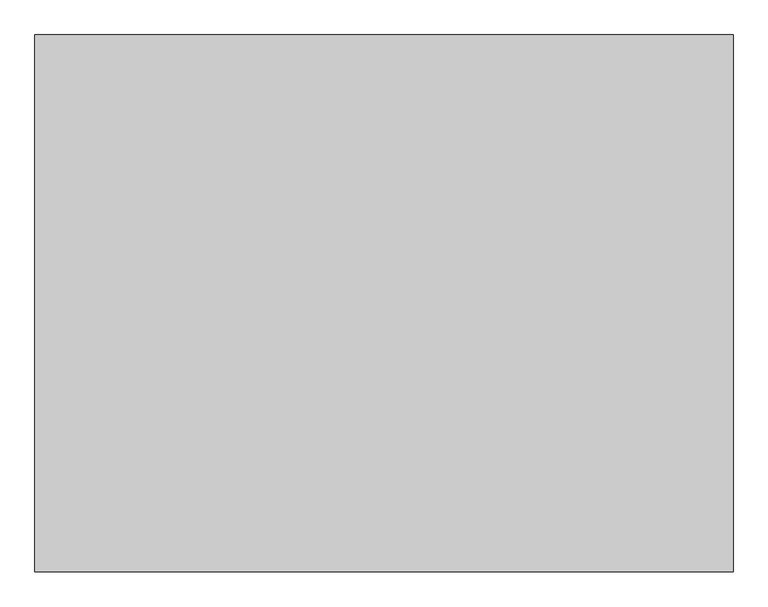
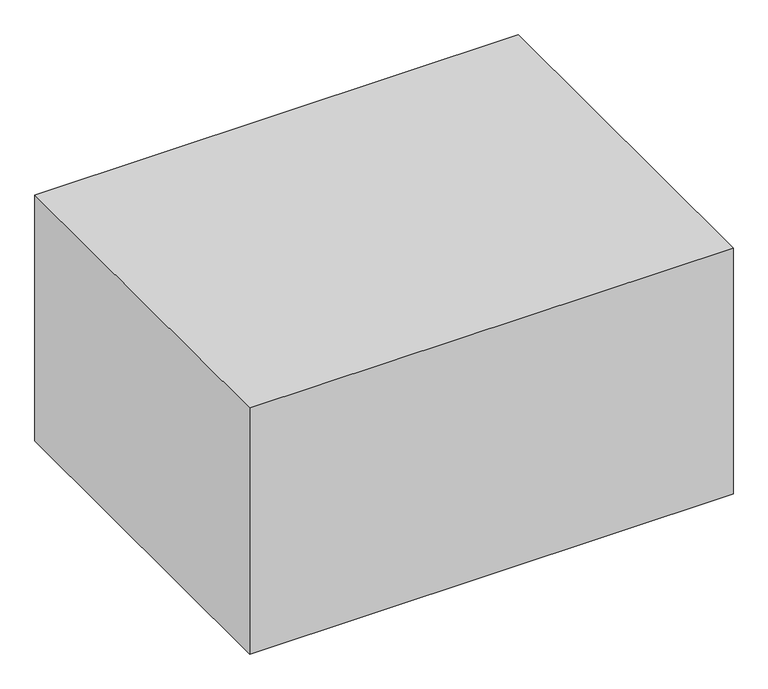
"""IFC4 building model written with IfcOpenShell, lengths in millimetres: proxy geometry, Space Planning Box_hec : Space Planning Box_hec."""

from ifc_helpers import new_model, si_unit, origin, origin_with_axes, place, context, project, spatial, polyline, outline, extrude, source, transform, mapped, element, save


def generic_models_249c6621(model_context):
    return source(origin(), model_context, "Body", "SweptSolid", [
        extrude(outline(polyline([(3250.0, 2500.0), (3250.0, -2500.0), (-3250.0, -2500.0), (-3250.0, 2500.0), (3250.0, 2500.0)])), origin_with_axes(), (0.0, 0.0, 1.0), 3500.0),
    ])


if __name__ == "__main__":
    model = new_model("IFC4")
    model_context = context("Model", 3, world=origin())
    ifc_project = project(units=[si_unit("LENGTHUNIT", "METRE", prefix="MILLI")], contexts=[model_context])
    site = spatial("IfcSite", under=ifc_project)
    building = spatial("IfcBuilding", under=site)
    placement = place(None, origin())
    generic_models_shape = generic_models_249c6621(model_context)
    element("IfcBuildingElementProxy", 1, Name="Space Planning Box_hec : Space Planning Box_hec", ObjectType="Space Planning Box_hec : Space Planning Box_hec", at=placement, inside=building, context=model_context, shape_type="MappedRepresentation", body=[
        mapped(generic_models_shape, transform((0.0, 0.0, 0.0), x_axis=(1.0, 0.0, 0.0), y_axis=(0.0, 1.0, 0.0), z_axis=(0.0, 0.0, 1.0))),
    ])
    save(model, "model.ifc")

# Revit data of these elements
# Type "Space Planning Box_hec : Space Planning Box_hec"
#   Type Comments = "..."
#   Room Name [instance default] = "?"
#   Interior Finish [instance default] = ""
#   Exterior Finish [instance default] = ""
#   Department [instance default] = ""
#   Assembly Code = "..."
#   ceiling height [instance default] = 0
#   Width [instance default] = 1524 mm
#   Program Area [instance default] = 0.00 m²
#   Length [instance default] = 1524 mm
#   Height [instance default] = 1524 mm
#   Area [instance default] = 2.32258 m²
#   Fill Color [instance default] = Cyan
#   Default Elevation = 0
# Element 1 (IfcBuildingElementProxy, "Space Planning Box_hec : Space Planning Box_hec")
#   Room Name = "Office-1"
#   Exterior Finish = "RF1..N/A,,EW2..N/A..N/A"
#   Department = "AR"
#   Width = 6500 mm
#   Program Area = 32.50 m²
#   Length = 5000 mm
#   Height = 3500 mm
#   Area = 32.50 m²
#   Materials on its faces: "Cyan"
# Materials
#   "Cyan": class "Generic", colour RGB 0 255 255, transparency 0.2, Cost = 0
